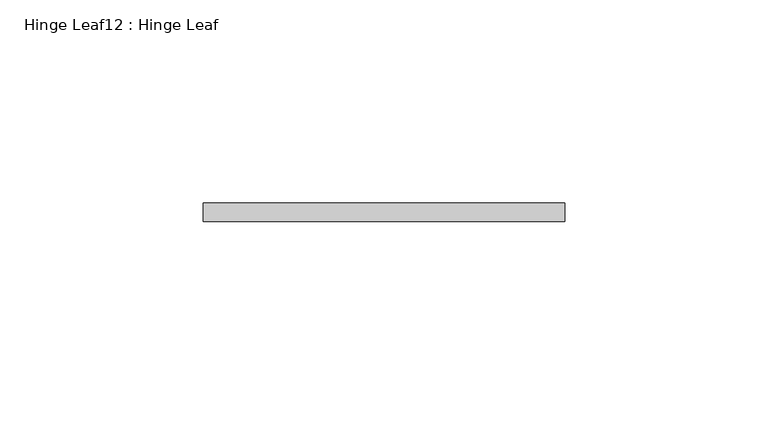
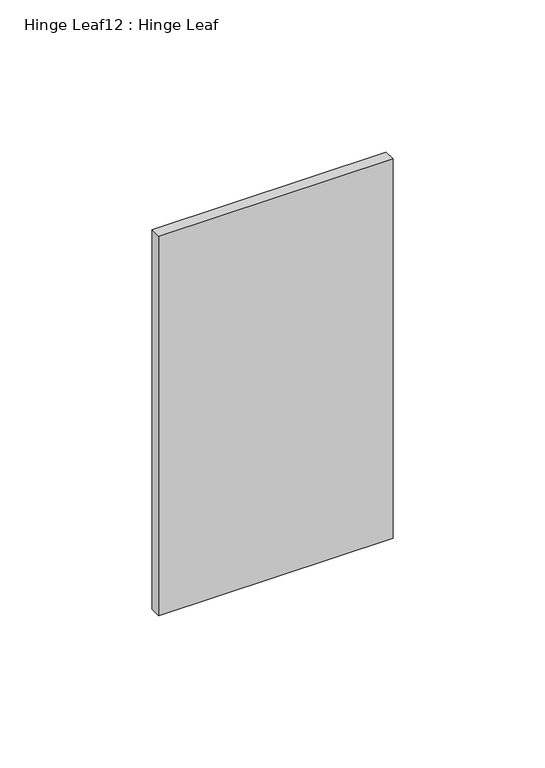
"""IFC4 building model written with IfcOpenShell, lengths in millimetres: proxy geometry, Hinge Leaf12 : Hinge Leaf."""

from ifc_helpers import new_model, si_unit, frame, origin, place, context, project, spatial, polyline, outline, extrude, source, transform, mapped, element, save


def hinge_leaf12_hinge_leaf_05c7f3a5(model_context):
    return source(origin(), model_context, "Body", "SweptSolid", [
        extrude(outline(polyline([(587327.7934739, -533980.5883841), (587327.7934739, -533976.0163841), (587416.6934739, -533976.0163841), (587416.6934739, -533980.5883841), (587327.7934739, -533980.5883841)])), frame((0.0, 0.0, 1123.95), z_axis=(0.0, 0.0, 1.0), x_axis=(1.0, 0.0, 0.0)), (0.0, 0.0, 1.0), 152.4),
    ])


if __name__ == "__main__":
    model = new_model("IFC4")
    model_context = context("Model", 3, world=origin())
    ifc_project = project(units=[si_unit("LENGTHUNIT", "METRE", prefix="MILLI")], contexts=[model_context])
    site = spatial("IfcSite", under=ifc_project)
    building = spatial("IfcBuilding", under=site)
    placement = place(None, origin())
    hinge_leaf12_hinge_leaf_shape = hinge_leaf12_hinge_leaf_05c7f3a5(model_context)
    element("IfcBuildingElementProxy", 1, Name="Hinge Leaf12 : Hinge Leaf", ObjectType="Hinge Leaf12 : Hinge Leaf", at=placement, inside=building, context=model_context, shape_type="MappedRepresentation", body=[
        mapped(hinge_leaf12_hinge_leaf_shape, transform((0.0, 0.0, 0.0), x_axis=(1.0, 0.0, 0.0), y_axis=(0.0, 1.0, 0.0), z_axis=(0.0, 0.0, 1.0))),
    ])
    save(model, "model.ifc")

# Revit data of these elements
# Element 1 (IfcBuildingElementProxy, "Hinge Leaf12 : Hinge Leaf")
#   Materials on its faces: "6\"X6\" WELD-ON STL BUTT HINGE"
# Materials
#   "6\"X6\" WELD-ON STL BUTT HINGE": class "Metal", colour RGB 189 187 185, transparency 0, Description = "Carbon steel", Cost = 0
